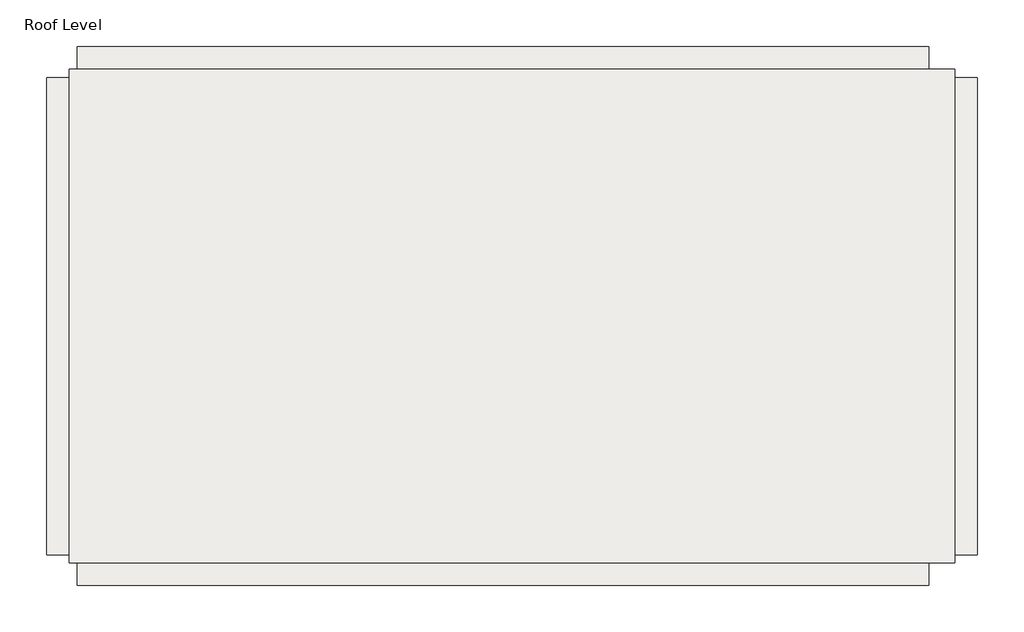
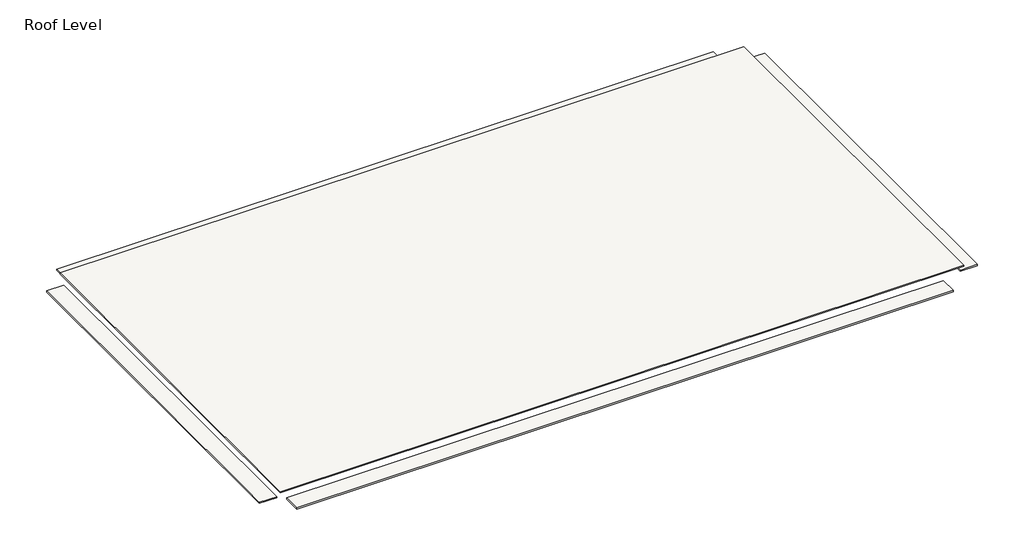
# One storey: 5 roofs.
"""IFC4 building model written with IfcOpenShell, lengths in millimetres."""

import ifcopenshell
import ifcopenshell.guid

model = None  # the IFC model being written
_history = None  # IfcOwnerHistory: only IFC2X3 demands one
_inside = {}  # id of a spatial element -> (the spatial element, [elements in it])
_under = {}  # id of a project, library or spatial element -> (it, [spatial elements below it])
_declared = {}  # id of a project -> (the project, [libraries it declares])
_typed = {}  # id of a type object -> (the type object, [elements of that type])
_made_of = {}  # id of a material, layer set ... -> (it, [elements and type objects made of it])


def new_model(schema):
    """Start an empty IFC model of exactly this schema.

    Asked for "IFC4X3", IfcOpenShell would pick the latest addendum, in which some entities
    have other attributes; the version numbers below select the first issue.
    IFC2X3 requires an IfcOwnerHistory on every rooted entity: one is made here for all.
    """
    global model, _history
    if schema == "IFC4X3":
        model = ifcopenshell.file(schema_version=(4, 3, 0, 0))
    else:
        model = ifcopenshell.file(schema=schema)
    _inside.clear()
    _under.clear()
    _declared.clear()
    _typed.clear()
    _made_of.clear()
    _history = None
    if model.schema == "IFC2X3":
        org = make("IfcOrganization", Name="unknown")
        user = make(
            "IfcPersonAndOrganization",
            ThePerson=make("IfcPerson", FamilyName="unknown"),
            TheOrganization=org,
        )
        app = make(
            "IfcApplication",
            ApplicationDeveloper=org,
            Version="unknown",
            ApplicationFullName="unknown",
            ApplicationIdentifier="unknown",
        )
        _history = make(
            "IfcOwnerHistory",
            OwningUser=user,
            OwningApplication=app,
            ChangeAction="ADDED",
            CreationDate=0,
        )
    return model


def make(cls, **values):
    """One entity of the class cls with the attributes given. An attribute that is None is left unset."""
    return model.create_entity(
        cls, **{name: value for name, value in values.items() if value is not None}
    )


def rooted(cls, **values):
    """An entity with a GlobalId (a new one), such as an element, a storey or a relation."""
    return make(cls, GlobalId=ifcopenshell.guid.new(), OwnerHistory=_history, **values)


def si_unit(unit_type, name, prefix=None):
    """IfcSIUnit, for example si_unit("LENGTHUNIT", "METRE", prefix="MILLI")."""
    return make("IfcSIUnit", UnitType=unit_type, Prefix=prefix, Name=name)


def assignment(units):
    """IfcUnitAssignment: the units of a project."""
    return None if units is None else make("IfcUnitAssignment", Units=units)


def point(xyz):
    """IfcCartesianPoint."""
    return None if xyz is None else make("IfcCartesianPoint", Coordinates=xyz)


def direction(xyz):
    """IfcDirection."""
    return None if xyz is None else make("IfcDirection", DirectionRatios=xyz)


def frame(location, z_axis=None, x_axis=None):
    """IfcAxis2Placement3D, a coordinate frame: its origin and axes. An axis left out is left unset."""
    return make(
        "IfcAxis2Placement3D",
        Location=point(location),
        Axis=direction(z_axis),
        RefDirection=direction(x_axis),
    )


def origin():
    """The frame at (0, 0, 0) with its axes left unset."""
    return frame((0.0, 0.0, 0.0))


def place(relative_to, where):
    """IfcLocalPlacement: puts the frame where relative to a parent placement (None: the world)."""
    return make(
        "IfcLocalPlacement", PlacementRelTo=relative_to, RelativePlacement=where
    )


def context(
    kind, dimensions, precision=None, world=None, true_north=None, identifier=None
):
    """IfcGeometricRepresentationContext, for example the 3D "Model" context."""
    return make(
        "IfcGeometricRepresentationContext",
        ContextIdentifier=identifier,
        ContextType=kind,
        CoordinateSpaceDimension=dimensions,
        Precision=precision,
        WorldCoordinateSystem=world,
        TrueNorth=true_north,
    )


def project(units=None, contexts=None):
    """IfcProject with its units and contexts."""
    return rooted(
        "IfcProject",
        Name="project",
        RepresentationContexts=contexts,
        UnitsInContext=assignment(units),
    )


def spatial(cls, under=None, at=None, **own):
    """A site, building, storey or space (cls), placed at a placement, below another one or the project."""
    s = rooted(cls, ObjectPlacement=at, **own)
    if under is not None:
        _under.setdefault(under.id(), (under, []))[1].append(s)
    return s


def polyline(points):
    """IfcPolyline through the points."""
    return make("IfcPolyline", Points=[point(p) for p in points])


def outline(outer, holes=None, kind="AREA"):
    """IfcArbitraryClosedProfileDef: a profile drawn as a closed curve; with holes, ...WithVoids."""
    if holes is None:
        return make("IfcArbitraryClosedProfileDef", ProfileType=kind, OuterCurve=outer)
    return make(
        "IfcArbitraryProfileDefWithVoids",
        ProfileType=kind,
        OuterCurve=outer,
        InnerCurves=holes,
    )


def extrude(swept, where, along, depth):
    """IfcExtrudedAreaSolid: the profile swept, set in the frame where, extruded along a direction by depth."""
    return make(
        "IfcExtrudedAreaSolid",
        SweptArea=swept,
        Position=where,
        ExtrudedDirection=direction(along),
        Depth=depth,
    )


def shape(context_of_items, identifier, shape_type, items):
    """IfcShapeRepresentation: the items that make up one representation, for example the "Body"."""
    return make(
        "IfcShapeRepresentation",
        ContextOfItems=context_of_items,
        RepresentationIdentifier=identifier,
        RepresentationType=shape_type,
        Items=items,
    )


def made_of(thing, what):
    """Note that an element or type object is made of a material, layer set ...; save() writes the relation."""
    if what is not None:
        _made_of.setdefault(what.id(), (what, []))[1].append(thing)
    return thing


def element(
    cls,
    number,
    at=None,
    inside=None,
    cuts=None,
    type_object=None,
    material=None,
    context=None,
    identifier="Body",
    shape_type=None,
    held_by="IfcProductDefinitionShape",
    body=None,
    shapes=None,
    **own,
):
    """One element of the class cls, such as IfcWall. Its Tag is "e" and its number.

    at: its placement. inside: the storey or other place that contains it. cuts: it is an
    opening in that element (IfcRelVoidsElement). A single representation is given by context,
    identifier, shape_type and body (its items); several are given by shapes. held_by: the class
    of the entity that holds the representations. save() writes the other relations.
    """
    e = rooted(cls, Tag="e%d" % number, ObjectPlacement=at, **own)
    if body is not None:
        shapes = [shape(context, identifier, shape_type, body)]
    if shapes is not None:
        e.Representation = make(held_by, Representations=shapes)
    if inside is not None:
        _inside.setdefault(inside.id(), (inside, []))[1].append(e)
    if cuts is not None:
        rooted(
            "IfcRelVoidsElement", RelatingBuildingElement=cuts, RelatedOpeningElement=e
        )
    if type_object is not None:
        _typed.setdefault(type_object.id(), (type_object, []))[1].append(e)
    return made_of(e, material)


def aggregate(whole, parts):
    """IfcRelAggregates: a whole, such as a stair, and the parts it consists of."""
    return rooted("IfcRelAggregates", RelatingObject=whole, RelatedObjects=parts)


def save(model, path):
    """Write the relations noted so far, then the file.

    IfcRelAggregates (storeys below a building ...), IfcRelContainedInSpatialStructure (elements
    in a storey), IfcRelDefinesByType, IfcRelAssociatesMaterial and IfcRelDeclares: one each for
    every whole, place, type object, material and project.
    """
    for whole, parts in _under.values():
        aggregate(whole, parts)
    for where, things in _inside.values():
        rooted(
            "IfcRelContainedInSpatialStructure",
            RelatedElements=things,
            RelatingStructure=where,
        )
    for kind, things in _typed.values():
        rooted("IfcRelDefinesByType", RelatedObjects=things, RelatingType=kind)
    for what, things in _made_of.values():
        rooted("IfcRelAssociatesMaterial", RelatedObjects=things, RelatingMaterial=what)
    for by, libraries in _declared.values():
        rooted("IfcRelDeclares", RelatingContext=by, RelatedDefinitions=libraries)
    model.write(path)


model = new_model("IFC4")

# Units and contexts
model_context = context("Model", 3, world=origin())
ifc_project = project(units=[si_unit("LENGTHUNIT", "METRE", prefix="MILLI")], contexts=[model_context])

# Site, building, storey
site = spatial("IfcSite", under=ifc_project)
building = spatial("IfcBuilding", under=site)
storey = spatial("IfcBuildingStorey", under=building, Name="Roof Level", Elevation=7924.8)

# Roofs
placement = place(None, origin())
element("IfcRoof", 1, ObjectType="Shading devices - 50mm", at=placement, inside=storey, context=model_context, shape_type="SweptSolid", body=[
    extrude(outline(polyline([(1746.464681, -4095.4197783), (28246.464681, -4095.4197783), (28246.464681, -4795.4197783), (1746.464681, -4795.4197783), (1746.464681, -4095.4197783)])), frame((0.0, 0.0, 7562.4), z_axis=(0.0, 0.0, 1.0), x_axis=(1.0, 0.0, 0.0)), (0.0, 0.0, 1.0), 50.0),
])
element("IfcRoof", 2, ObjectType="Shading devices - 50mm", at=placement, inside=storey, context=model_context, shape_type="SweptSolid", body=[
    extrude(outline(polyline([(29068.464681, 11030.5802217), (29768.464681, 11030.5802217), (29768.464681, -3843.0197783), (29068.464681, -3843.0197783), (29068.464681, 11030.5802217)])), frame((0.0, 0.0, 7562.4), z_axis=(0.0, 0.0, 1.0), x_axis=(1.0, 0.0, 0.0)), (0.0, 0.0, 1.0), 50.0),
])
element("IfcRoof", 3, ObjectType="Shading devices - 50mm", at=placement, inside=storey, context=model_context, shape_type="SweptSolid", body=[
    extrude(outline(polyline([(28246.464681, 11296.9802217), (1746.464681, 11296.9802217), (1746.464681, 11996.9802217), (28246.464681, 11996.9802217), (28246.464681, 11296.9802217)])), frame((0.0, 0.0, 7562.4), z_axis=(0.0, 0.0, 1.0), x_axis=(1.0, 0.0, 0.0)), (0.0, 0.0, 1.0), 50.0),
])
element("IfcRoof", 4, ObjectType="Shading devices - 50mm", at=placement, inside=storey, context=model_context, shape_type="SweptSolid", body=[
    extrude(outline(polyline([(784.064681, 11030.5802217), (1484.064681, 11030.5802217), (1484.064681, -3843.0197783), (784.064681, -3843.0197783), (784.064681, 11030.5802217)])), frame((0.0, 0.0, 7562.4), z_axis=(0.0, 0.0, 1.0), x_axis=(1.0, 0.0, 0.0)), (0.0, 0.0, 1.0), 50.0),
])
element("IfcRoof", 5, ObjectType="Shading devices - 50mm", at=placement, inside=storey, context=model_context, shape_type="SweptSolid", body=[
    extrude(outline(polyline([(1484.064681, 11296.9802217), (29068.464681, 11296.9802217), (29068.464681, -4095.4197783), (1484.064681, -4095.4197783), (1484.064681, 11296.9802217)])), frame((0.0, 0.0, 7924.8), z_axis=(0.0, 0.0, 1.0), x_axis=(1.0, 0.0, 0.0)), (0.0, 0.0, 1.0), 50.0),
])

save(model, "model.ifc")

# Revit data of these elements
# Type "Shading devices - 50mm"
#   Layers, outside or top first: 50 mm no material (function 1)
# Elements 1, 2, 3, 4 (IfcRoof, "Shading devices - 50mm")
#   built-in parameter 1001705 = 24.9751 (stored number, unit not read)
#   built-in parameter 1001701 = -1.18898 (stored number, unit not read)
#   built-in parameter 1001710 = 33615
#   Phase Created = New Construction
#   Materials on its faces: "Default Roof"
# Element 5 (IfcRoof, "Shading devices - 50mm")
#   built-in parameter 1001705 = 26.164 (stored number, unit not read)
#   built-in parameter 1001710 = 33615
#   Phase Created = New Construction
#   Materials on its faces: "Default Roof"
# Materials
#   "Default Roof": class "Miscellaneous", colour RGB 0 127 0, transparency 0, Cost = 0
